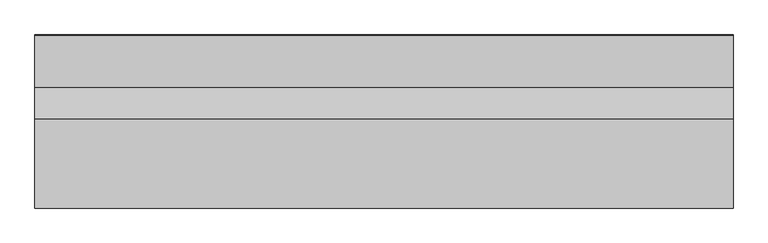
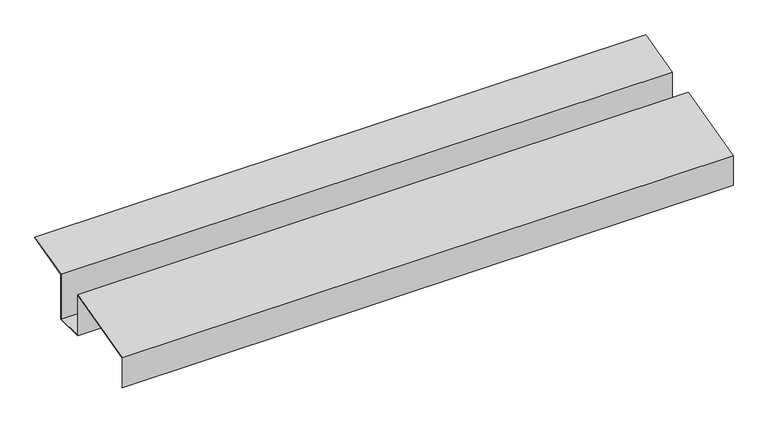
"""IFC4 building model written with IfcOpenShell, lengths in millimetres: proxy geometry, Gutter Adherance Membrane : Gutter Adherance Membrane."""

import ifcopenshell
import ifcopenshell.guid

model = None  # the IFC model being written
_history = None  # IfcOwnerHistory: only IFC2X3 demands one
_inside = {}  # id of a spatial element -> (the spatial element, [elements in it])
_under = {}  # id of a project, library or spatial element -> (it, [spatial elements below it])
_declared = {}  # id of a project -> (the project, [libraries it declares])
_typed = {}  # id of a type object -> (the type object, [elements of that type])
_made_of = {}  # id of a material, layer set ... -> (it, [elements and type objects made of it])


def new_model(schema):
    """Start an empty IFC model of exactly this schema.

    Asked for "IFC4X3", IfcOpenShell would pick the latest addendum, in which some entities
    have other attributes; the version numbers below select the first issue.
    IFC2X3 requires an IfcOwnerHistory on every rooted entity: one is made here for all.
    """
    global model, _history
    if schema == "IFC4X3":
        model = ifcopenshell.file(schema_version=(4, 3, 0, 0))
    else:
        model = ifcopenshell.file(schema=schema)
    _inside.clear()
    _under.clear()
    _declared.clear()
    _typed.clear()
    _made_of.clear()
    _history = None
    if model.schema == "IFC2X3":
        org = make("IfcOrganization", Name="unknown")
        user = make(
            "IfcPersonAndOrganization",
            ThePerson=make("IfcPerson", FamilyName="unknown"),
            TheOrganization=org,
        )
        app = make(
            "IfcApplication",
            ApplicationDeveloper=org,
            Version="unknown",
            ApplicationFullName="unknown",
            ApplicationIdentifier="unknown",
        )
        _history = make(
            "IfcOwnerHistory",
            OwningUser=user,
            OwningApplication=app,
            ChangeAction="ADDED",
            CreationDate=0,
        )
    return model


def make(cls, **values):
    """One entity of the class cls with the attributes given. An attribute that is None is left unset."""
    return model.create_entity(
        cls, **{name: value for name, value in values.items() if value is not None}
    )


def rooted(cls, **values):
    """An entity with a GlobalId (a new one), such as an element, a storey or a relation."""
    return make(cls, GlobalId=ifcopenshell.guid.new(), OwnerHistory=_history, **values)


def si_unit(unit_type, name, prefix=None):
    """IfcSIUnit, for example si_unit("LENGTHUNIT", "METRE", prefix="MILLI")."""
    return make("IfcSIUnit", UnitType=unit_type, Prefix=prefix, Name=name)


def assignment(units):
    """IfcUnitAssignment: the units of a project."""
    return None if units is None else make("IfcUnitAssignment", Units=units)


def point(xyz):
    """IfcCartesianPoint."""
    return None if xyz is None else make("IfcCartesianPoint", Coordinates=xyz)


def direction(xyz):
    """IfcDirection."""
    return None if xyz is None else make("IfcDirection", DirectionRatios=xyz)


def frame(location, z_axis=None, x_axis=None):
    """IfcAxis2Placement3D, a coordinate frame: its origin and axes. An axis left out is left unset."""
    return make(
        "IfcAxis2Placement3D",
        Location=point(location),
        Axis=direction(z_axis),
        RefDirection=direction(x_axis),
    )


def origin():
    """The frame at (0, 0, 0) with its axes left unset."""
    return frame((0.0, 0.0, 0.0))


def place(relative_to, where):
    """IfcLocalPlacement: puts the frame where relative to a parent placement (None: the world)."""
    return make(
        "IfcLocalPlacement", PlacementRelTo=relative_to, RelativePlacement=where
    )


def context(
    kind, dimensions, precision=None, world=None, true_north=None, identifier=None
):
    """IfcGeometricRepresentationContext, for example the 3D "Model" context."""
    return make(
        "IfcGeometricRepresentationContext",
        ContextIdentifier=identifier,
        ContextType=kind,
        CoordinateSpaceDimension=dimensions,
        Precision=precision,
        WorldCoordinateSystem=world,
        TrueNorth=true_north,
    )


def project(units=None, contexts=None):
    """IfcProject with its units and contexts."""
    return rooted(
        "IfcProject",
        Name="project",
        RepresentationContexts=contexts,
        UnitsInContext=assignment(units),
    )


def spatial(cls, under=None, at=None, **own):
    """A site, building, storey or space (cls), placed at a placement, below another one or the project."""
    s = rooted(cls, ObjectPlacement=at, **own)
    if under is not None:
        _under.setdefault(under.id(), (under, []))[1].append(s)
    return s


def polyline(points):
    """IfcPolyline through the points."""
    return make("IfcPolyline", Points=[point(p) for p in points])


def outline(outer, holes=None, kind="AREA"):
    """IfcArbitraryClosedProfileDef: a profile drawn as a closed curve; with holes, ...WithVoids."""
    if holes is None:
        return make("IfcArbitraryClosedProfileDef", ProfileType=kind, OuterCurve=outer)
    return make(
        "IfcArbitraryProfileDefWithVoids",
        ProfileType=kind,
        OuterCurve=outer,
        InnerCurves=holes,
    )


def extrude(swept, where, along, depth):
    """IfcExtrudedAreaSolid: the profile swept, set in the frame where, extruded along a direction by depth."""
    return make(
        "IfcExtrudedAreaSolid",
        SweptArea=swept,
        Position=where,
        ExtrudedDirection=direction(along),
        Depth=depth,
    )


def shape(context_of_items, identifier, shape_type, items):
    """IfcShapeRepresentation: the items that make up one representation, for example the "Body"."""
    return make(
        "IfcShapeRepresentation",
        ContextOfItems=context_of_items,
        RepresentationIdentifier=identifier,
        RepresentationType=shape_type,
        Items=items,
    )


def source(mapping_origin, context_of_items, identifier, shape_type, items):
    """IfcRepresentationMap: a shape defined once, which mapped items show again and again."""
    return make(
        "IfcRepresentationMap",
        MappingOrigin=mapping_origin,
        MappedRepresentation=shape(context_of_items, identifier, shape_type, items),
    )


def transform(
    local_origin,
    x_axis=None,
    y_axis=None,
    z_axis=None,
    scale=None,
    scale2=None,
    scale3=None,
    uniform=True,
):
    """IfcCartesianTransformationOperator3D, or its non-uniform kind. x_axis, y_axis, z_axis: its Axis1, 2, 3."""
    if uniform:
        return make(
            "IfcCartesianTransformationOperator3D",
            Axis1=direction(x_axis),
            Axis2=direction(y_axis),
            LocalOrigin=point(local_origin),
            Scale=scale,
            Axis3=direction(z_axis),
        )
    return make(
        "IfcCartesianTransformationOperator3DnonUniform",
        Axis1=direction(x_axis),
        Axis2=direction(y_axis),
        LocalOrigin=point(local_origin),
        Scale=scale,
        Axis3=direction(z_axis),
        Scale2=scale2,
        Scale3=scale3,
    )


def mapped(mapping_source, mapping_target):
    """IfcMappedItem: shows the shape of a source again, moved by a transform."""
    return make(
        "IfcMappedItem", MappingSource=mapping_source, MappingTarget=mapping_target
    )


def made_of(thing, what):
    """Note that an element or type object is made of a material, layer set ...; save() writes the relation."""
    if what is not None:
        _made_of.setdefault(what.id(), (what, []))[1].append(thing)
    return thing


def element(
    cls,
    number,
    at=None,
    inside=None,
    cuts=None,
    type_object=None,
    material=None,
    context=None,
    identifier="Body",
    shape_type=None,
    held_by="IfcProductDefinitionShape",
    body=None,
    shapes=None,
    **own,
):
    """One element of the class cls, such as IfcWall. Its Tag is "e" and its number.

    at: its placement. inside: the storey or other place that contains it. cuts: it is an
    opening in that element (IfcRelVoidsElement). A single representation is given by context,
    identifier, shape_type and body (its items); several are given by shapes. held_by: the class
    of the entity that holds the representations. save() writes the other relations.
    """
    e = rooted(cls, Tag="e%d" % number, ObjectPlacement=at, **own)
    if body is not None:
        shapes = [shape(context, identifier, shape_type, body)]
    if shapes is not None:
        e.Representation = make(held_by, Representations=shapes)
    if inside is not None:
        _inside.setdefault(inside.id(), (inside, []))[1].append(e)
    if cuts is not None:
        rooted(
            "IfcRelVoidsElement", RelatingBuildingElement=cuts, RelatedOpeningElement=e
        )
    if type_object is not None:
        _typed.setdefault(type_object.id(), (type_object, []))[1].append(e)
    return made_of(e, material)


def aggregate(whole, parts):
    """IfcRelAggregates: a whole, such as a stair, and the parts it consists of."""
    return rooted("IfcRelAggregates", RelatingObject=whole, RelatedObjects=parts)


def save(model, path):
    """Write the relations noted so far, then the file.

    IfcRelAggregates (storeys below a building ...), IfcRelContainedInSpatialStructure (elements
    in a storey), IfcRelDefinesByType, IfcRelAssociatesMaterial and IfcRelDeclares: one each for
    every whole, place, type object, material and project.
    """
    for whole, parts in _under.values():
        aggregate(whole, parts)
    for where, things in _inside.values():
        rooted(
            "IfcRelContainedInSpatialStructure",
            RelatedElements=things,
            RelatingStructure=where,
        )
    for kind, things in _typed.values():
        rooted("IfcRelDefinesByType", RelatedObjects=things, RelatingType=kind)
    for what, things in _made_of.values():
        rooted("IfcRelAssociatesMaterial", RelatedObjects=things, RelatingMaterial=what)
    for by, libraries in _declared.values():
        rooted("IfcRelDeclares", RelatingContext=by, RelatedDefinitions=libraries)
    model.write(path)


def generic_models_17db74e9(model_context):
    return source(origin(), model_context, "Body", "SweptSolid", [
        extrude(outline(polyline([(-5246.5306641, 42821.4572967), (-5246.5306641, 42666.75625), (-5342.2945313, 42666.75625), (-5342.2945313, 42807.3923035), (-5593.0479292, 42742.5820053), (-5593.0479292, 42640.9820053), (-5594.6354292, 42640.9820053), (-5594.6354292, 42743.811364), (-5340.7070313, 42809.4422799), (-5340.7070313, 42668.34375), (-5248.1181641, 42668.34375), (-5248.1181641, 42822.6866554), (-5099.0584144, 42861.21298), (-5098.6611598, 42859.6759878), (-5246.5306641, 42821.4572967)])), frame((12382.7678845, 0.0, 0.0), z_axis=(1.0, 0.0, 0.0), x_axis=(0.0, 1.0, 0.0)), (0.0, 0.0, 1.0), 2000.25),
    ])


if __name__ == "__main__":
    model = new_model("IFC4")
    model_context = context("Model", 3, world=origin())
    ifc_project = project(units=[si_unit("LENGTHUNIT", "METRE", prefix="MILLI")], contexts=[model_context])
    site = spatial("IfcSite", under=ifc_project)
    building = spatial("IfcBuilding", under=site)
    placement = place(None, origin())
    generic_models_shape = generic_models_17db74e9(model_context)
    element("IfcBuildingElementProxy", 1, Name="Gutter Adherance Membrane : Gutter Adherance Membrane", ObjectType="Gutter Adherance Membrane : Gutter Adherance Membrane", at=placement, inside=building, context=model_context, shape_type="MappedRepresentation", body=[
        mapped(generic_models_shape, transform((0.0, 0.0, 0.0), x_axis=(1.0, 0.0, 0.0), y_axis=(0.0, 1.0, 0.0), z_axis=(0.0, 0.0, 1.0))),
    ])
    save(model, "model.ifc")

# Revit data of these elements
# Type "Gutter Adherance Membrane : Gutter Adherance Membrane"
#   NameOverride = "Gutter Adherance Membrane"
# Element 1 (IfcBuildingElementProxy, "Gutter Adherance Membrane : Gutter Adherance Membrane")
#   Materials on its faces: "SELF ADHERED MEMBRANE W/ END DAMS WHERE POSSIBLE"
# Materials
#   "SELF ADHERED MEMBRANE W/ END DAMS WHERE POSSIBLE": class "Unassigned", colour RGB 255 255 127, transparency 0
